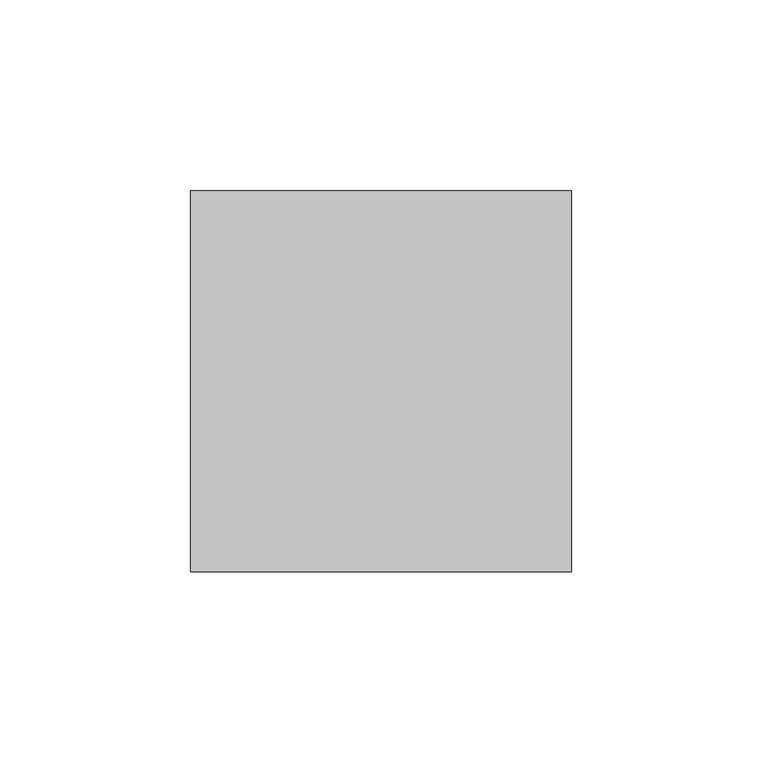
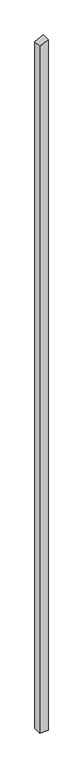
"""IFC4 building model written with IfcOpenShell, lengths in millimetres: column geometry, Holzstütze 158656 : Holzstütze 158656."""

import ifcopenshell
import ifcopenshell.guid

model = None  # the IFC model being written
_history = None  # IfcOwnerHistory: only IFC2X3 demands one
_inside = {}  # id of a spatial element -> (the spatial element, [elements in it])
_under = {}  # id of a project, library or spatial element -> (it, [spatial elements below it])
_declared = {}  # id of a project -> (the project, [libraries it declares])
_typed = {}  # id of a type object -> (the type object, [elements of that type])
_made_of = {}  # id of a material, layer set ... -> (it, [elements and type objects made of it])


def new_model(schema):
    """Start an empty IFC model of exactly this schema.

    Asked for "IFC4X3", IfcOpenShell would pick the latest addendum, in which some entities
    have other attributes; the version numbers below select the first issue.
    IFC2X3 requires an IfcOwnerHistory on every rooted entity: one is made here for all.
    """
    global model, _history
    if schema == "IFC4X3":
        model = ifcopenshell.file(schema_version=(4, 3, 0, 0))
    else:
        model = ifcopenshell.file(schema=schema)
    _inside.clear()
    _under.clear()
    _declared.clear()
    _typed.clear()
    _made_of.clear()
    _history = None
    if model.schema == "IFC2X3":
        org = make("IfcOrganization", Name="unknown")
        user = make(
            "IfcPersonAndOrganization",
            ThePerson=make("IfcPerson", FamilyName="unknown"),
            TheOrganization=org,
        )
        app = make(
            "IfcApplication",
            ApplicationDeveloper=org,
            Version="unknown",
            ApplicationFullName="unknown",
            ApplicationIdentifier="unknown",
        )
        _history = make(
            "IfcOwnerHistory",
            OwningUser=user,
            OwningApplication=app,
            ChangeAction="ADDED",
            CreationDate=0,
        )
    return model


def make(cls, **values):
    """One entity of the class cls with the attributes given. An attribute that is None is left unset."""
    return model.create_entity(
        cls, **{name: value for name, value in values.items() if value is not None}
    )


def rooted(cls, **values):
    """An entity with a GlobalId (a new one), such as an element, a storey or a relation."""
    return make(cls, GlobalId=ifcopenshell.guid.new(), OwnerHistory=_history, **values)


def si_unit(unit_type, name, prefix=None):
    """IfcSIUnit, for example si_unit("LENGTHUNIT", "METRE", prefix="MILLI")."""
    return make("IfcSIUnit", UnitType=unit_type, Prefix=prefix, Name=name)


def assignment(units):
    """IfcUnitAssignment: the units of a project."""
    return None if units is None else make("IfcUnitAssignment", Units=units)


def point(xyz):
    """IfcCartesianPoint."""
    return None if xyz is None else make("IfcCartesianPoint", Coordinates=xyz)


def direction(xyz):
    """IfcDirection."""
    return None if xyz is None else make("IfcDirection", DirectionRatios=xyz)


def frame(location, z_axis=None, x_axis=None):
    """IfcAxis2Placement3D, a coordinate frame: its origin and axes. An axis left out is left unset."""
    return make(
        "IfcAxis2Placement3D",
        Location=point(location),
        Axis=direction(z_axis),
        RefDirection=direction(x_axis),
    )


def origin():
    """The frame at (0, 0, 0) with its axes left unset."""
    return frame((0.0, 0.0, 0.0))


def place(relative_to, where):
    """IfcLocalPlacement: puts the frame where relative to a parent placement (None: the world)."""
    return make(
        "IfcLocalPlacement", PlacementRelTo=relative_to, RelativePlacement=where
    )


def context(
    kind, dimensions, precision=None, world=None, true_north=None, identifier=None
):
    """IfcGeometricRepresentationContext, for example the 3D "Model" context."""
    return make(
        "IfcGeometricRepresentationContext",
        ContextIdentifier=identifier,
        ContextType=kind,
        CoordinateSpaceDimension=dimensions,
        Precision=precision,
        WorldCoordinateSystem=world,
        TrueNorth=true_north,
    )


def project(units=None, contexts=None):
    """IfcProject with its units and contexts."""
    return rooted(
        "IfcProject",
        Name="project",
        RepresentationContexts=contexts,
        UnitsInContext=assignment(units),
    )


def spatial(cls, under=None, at=None, **own):
    """A site, building, storey or space (cls), placed at a placement, below another one or the project."""
    s = rooted(cls, ObjectPlacement=at, **own)
    if under is not None:
        _under.setdefault(under.id(), (under, []))[1].append(s)
    return s


def polyline(points):
    """IfcPolyline through the points."""
    return make("IfcPolyline", Points=[point(p) for p in points])


def outline(outer, holes=None, kind="AREA"):
    """IfcArbitraryClosedProfileDef: a profile drawn as a closed curve; with holes, ...WithVoids."""
    if holes is None:
        return make("IfcArbitraryClosedProfileDef", ProfileType=kind, OuterCurve=outer)
    return make(
        "IfcArbitraryProfileDefWithVoids",
        ProfileType=kind,
        OuterCurve=outer,
        InnerCurves=holes,
    )


def extrude(swept, where, along, depth):
    """IfcExtrudedAreaSolid: the profile swept, set in the frame where, extruded along a direction by depth."""
    return make(
        "IfcExtrudedAreaSolid",
        SweptArea=swept,
        Position=where,
        ExtrudedDirection=direction(along),
        Depth=depth,
    )


def shape(context_of_items, identifier, shape_type, items):
    """IfcShapeRepresentation: the items that make up one representation, for example the "Body"."""
    return make(
        "IfcShapeRepresentation",
        ContextOfItems=context_of_items,
        RepresentationIdentifier=identifier,
        RepresentationType=shape_type,
        Items=items,
    )


def source(mapping_origin, context_of_items, identifier, shape_type, items):
    """IfcRepresentationMap: a shape defined once, which mapped items show again and again."""
    return make(
        "IfcRepresentationMap",
        MappingOrigin=mapping_origin,
        MappedRepresentation=shape(context_of_items, identifier, shape_type, items),
    )


def transform(
    local_origin,
    x_axis=None,
    y_axis=None,
    z_axis=None,
    scale=None,
    scale2=None,
    scale3=None,
    uniform=True,
):
    """IfcCartesianTransformationOperator3D, or its non-uniform kind. x_axis, y_axis, z_axis: its Axis1, 2, 3."""
    if uniform:
        return make(
            "IfcCartesianTransformationOperator3D",
            Axis1=direction(x_axis),
            Axis2=direction(y_axis),
            LocalOrigin=point(local_origin),
            Scale=scale,
            Axis3=direction(z_axis),
        )
    return make(
        "IfcCartesianTransformationOperator3DnonUniform",
        Axis1=direction(x_axis),
        Axis2=direction(y_axis),
        LocalOrigin=point(local_origin),
        Scale=scale,
        Axis3=direction(z_axis),
        Scale2=scale2,
        Scale3=scale3,
    )


def mapped(mapping_source, mapping_target):
    """IfcMappedItem: shows the shape of a source again, moved by a transform."""
    return make(
        "IfcMappedItem", MappingSource=mapping_source, MappingTarget=mapping_target
    )


def made_of(thing, what):
    """Note that an element or type object is made of a material, layer set ...; save() writes the relation."""
    if what is not None:
        _made_of.setdefault(what.id(), (what, []))[1].append(thing)
    return thing


def element(
    cls,
    number,
    at=None,
    inside=None,
    cuts=None,
    type_object=None,
    material=None,
    context=None,
    identifier="Body",
    shape_type=None,
    held_by="IfcProductDefinitionShape",
    body=None,
    shapes=None,
    **own,
):
    """One element of the class cls, such as IfcWall. Its Tag is "e" and its number.

    at: its placement. inside: the storey or other place that contains it. cuts: it is an
    opening in that element (IfcRelVoidsElement). A single representation is given by context,
    identifier, shape_type and body (its items); several are given by shapes. held_by: the class
    of the entity that holds the representations. save() writes the other relations.
    """
    e = rooted(cls, Tag="e%d" % number, ObjectPlacement=at, **own)
    if body is not None:
        shapes = [shape(context, identifier, shape_type, body)]
    if shapes is not None:
        e.Representation = make(held_by, Representations=shapes)
    if inside is not None:
        _inside.setdefault(inside.id(), (inside, []))[1].append(e)
    if cuts is not None:
        rooted(
            "IfcRelVoidsElement", RelatingBuildingElement=cuts, RelatedOpeningElement=e
        )
    if type_object is not None:
        _typed.setdefault(type_object.id(), (type_object, []))[1].append(e)
    return made_of(e, material)


def aggregate(whole, parts):
    """IfcRelAggregates: a whole, such as a stair, and the parts it consists of."""
    return rooted("IfcRelAggregates", RelatingObject=whole, RelatedObjects=parts)


def save(model, path):
    """Write the relations noted so far, then the file.

    IfcRelAggregates (storeys below a building ...), IfcRelContainedInSpatialStructure (elements
    in a storey), IfcRelDefinesByType, IfcRelAssociatesMaterial and IfcRelDeclares: one each for
    every whole, place, type object, material and project.
    """
    for whole, parts in _under.values():
        aggregate(whole, parts)
    for where, things in _inside.values():
        rooted(
            "IfcRelContainedInSpatialStructure",
            RelatedElements=things,
            RelatingStructure=where,
        )
    for kind, things in _typed.values():
        rooted("IfcRelDefinesByType", RelatedObjects=things, RelatingType=kind)
    for what, things in _made_of.values():
        rooted("IfcRelAssociatesMaterial", RelatedObjects=things, RelatingMaterial=what)
    for by, libraries in _declared.values():
        rooted("IfcRelDeclares", RelatingContext=by, RelatedDefinitions=libraries)
    model.write(path)


def column_4b14859e(model_context):
    return source(origin(), model_context, "Body", "SweptSolid", [
        extrude(outline(polyline([(-500.0, 161027.7593015), (-500.0, 161127.7593015), (8297.1942973, 161127.7593015), (8246.2417524, 161027.7593015), (-500.0, 161027.7593015)])), frame((0.0, 47884.7962965, 0.0), z_axis=(0.0, 1.0, 0.0), x_axis=(0.0, 0.0, 1.0)), (0.0, 0.0, 1.0), 100.0),
    ])


if __name__ == "__main__":
    model = new_model("IFC4")
    model_context = context("Model", 3, world=origin())
    ifc_project = project(units=[si_unit("LENGTHUNIT", "METRE", prefix="MILLI")], contexts=[model_context])
    site = spatial("IfcSite", under=ifc_project)
    building = spatial("IfcBuilding", under=site)
    placement = place(None, origin())
    column_shape = column_4b14859e(model_context)
    element("IfcColumn", 1, ObjectType="Holzstütze 158656 : Holzstütze 158656", at=placement, inside=building, context=model_context, shape_type="MappedRepresentation", body=[
        mapped(column_shape, transform((0.0, 0.0, 0.0), x_axis=(1.0, 0.0, 0.0), y_axis=(0.0, 1.0, 0.0), z_axis=(0.0, 0.0, 1.0))),
    ])
    save(model, "model.ifc")

# Revit data of these elements
# Project information
#   Organization Name = "Organization Name"
#   Organization Description = "Organization Description"
#   Building Name = "Building Name"
#   IfcOrganization = "KURIARCHITEKTEN"
#   IfcApplicationVersion = "2023.1"
#   IfcApplicationName = "Allplan"
#   IfcSite GUID = "3xMs$kp1n46ejeur8tozco"
#   IfcBuilding GUID = "0i8UyhEYT3nv9HLlo1H2X7"
#   IfcProject GUID = "2x1YFttxr4OvBiL8xtaqeA"
#   NameOverride = "GEBÄUDE 1"
#   Project Issue Date = "Issue Date"
#   Project Status = "Project Status"
#   Client Name = "Client Name"
#   Project Address = "Enter address here\nAddress Line 2"
#   Project Name = "Project Name"
#   Project Number = "Project Number"
# Type "Holzstütze 158656 : Holzstütze 158656"
#   Abrechnungsart = "m"
#   Allright_Bauteil_ID = "0152St 0000143543"
#   Bezeichnung = "Holzstütze"
#   Codetext = "ST-HOLZ\\"
#   Gewerk = "Zimmer- und Holzbauarbeiten"
#   Material = "Holz"
#   Objektname = "Stütze"
#   NameOverride = "Holzstütze"
#   Reference = "Holzstütze"
#   Status = "NEW"
#   ThermalTransmittance = 0.0000 BTU/(h·ft²·°F)
#   Roll = 0.00°
#   Slope = 0.00°
#   2D Interaktion = yes
#   IsExternal = yes
#   LoadBearing = yes
# Element 1 (IfcColumn, "Holzstütze 158656 : Holzstütze 158656")
#   Materials on its faces: "holzschalung"
# Materials
#   "holzschalung": class "Unassigned", colour RGB 128 128 128, transparency 0
